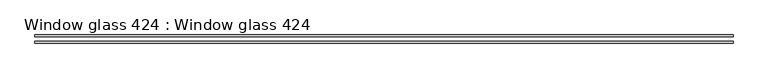
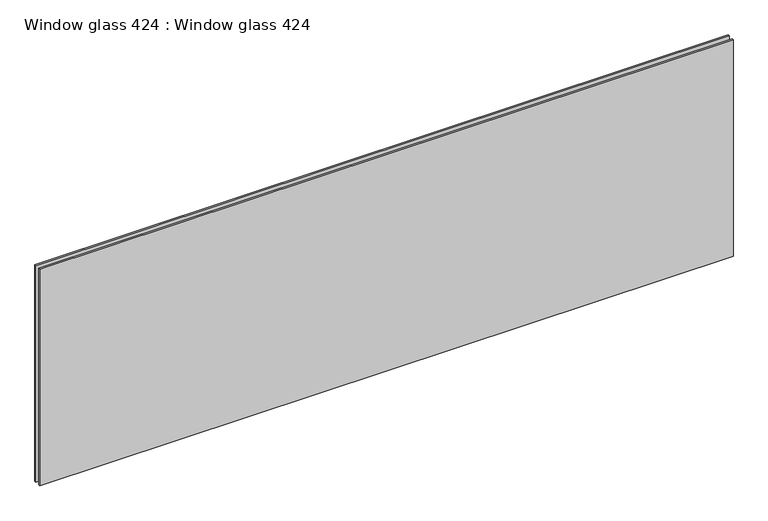
"""IFC4 building model written with IfcOpenShell, lengths in millimetres: proxy geometry, Window glass 424 : Window glass 424."""

from ifc_helpers import new_model, si_unit, frame, origin, place, context, project, spatial, polyline, outline, extrude, source, transform, mapped, element, save


def window_glass_424_window_glass_424_5d239823(model_context):
    return source(origin(), model_context, "Body", "SweptSolid", [
        extrude(outline(polyline([(3694.2883192, 10416.3326511), (3694.2883192, 10421.0951511), (5694.2883192, 10421.0951511), (5694.2883192, 10416.3326511), (3694.2883192, 10416.3326511)])), frame((0.0, 0.0, 40813.9765625), z_axis=(0.0, 0.0, 1.0), x_axis=(1.0, 0.0, 0.0)), (0.0, 0.0, 1.0), 660.4),
        extrude(outline(polyline([(3694.2883192, 10434.8746511), (3694.2883192, 10439.6371511), (5694.2883192, 10439.6371511), (5694.2883192, 10434.8746511), (3694.2883192, 10434.8746511)])), frame((0.0, 0.0, 40813.9765625), z_axis=(0.0, 0.0, 1.0), x_axis=(1.0, 0.0, 0.0)), (0.0, 0.0, 1.0), 660.4),
    ])


if __name__ == "__main__":
    model = new_model("IFC4")
    model_context = context("Model", 3, world=origin())
    ifc_project = project(units=[si_unit("LENGTHUNIT", "METRE", prefix="MILLI")], contexts=[model_context])
    site = spatial("IfcSite", under=ifc_project)
    building = spatial("IfcBuilding", under=site)
    placement = place(None, origin())
    window_glass_424_window_glass_424_shape = window_glass_424_window_glass_424_5d239823(model_context)
    element("IfcBuildingElementProxy", 1, Name="Window glass 424 : Window glass 424", ObjectType="Window glass 424 : Window glass 424", at=placement, inside=building, context=model_context, shape_type="MappedRepresentation", body=[
        mapped(window_glass_424_window_glass_424_shape, transform((0.0, 0.0, 0.0), x_axis=(1.0, 0.0, 0.0), y_axis=(0.0, 1.0, 0.0), z_axis=(0.0, 0.0, 1.0))),
    ])
    save(model, "model.ifc")

# Revit data of these elements
# Type "Window glass 424 : Window glass 424"
#   NameOverride = "Window glass"
# Element 1 (IfcBuildingElementProxy, "Window glass 424 : Window glass 424")
#   Materials on its faces: "1\"  INSULATED GLAZING"
# Materials
#   "1\"  INSULATED GLAZING": class "Unassigned", colour RGB 146 199 212, transparency 0, Cost = 0
